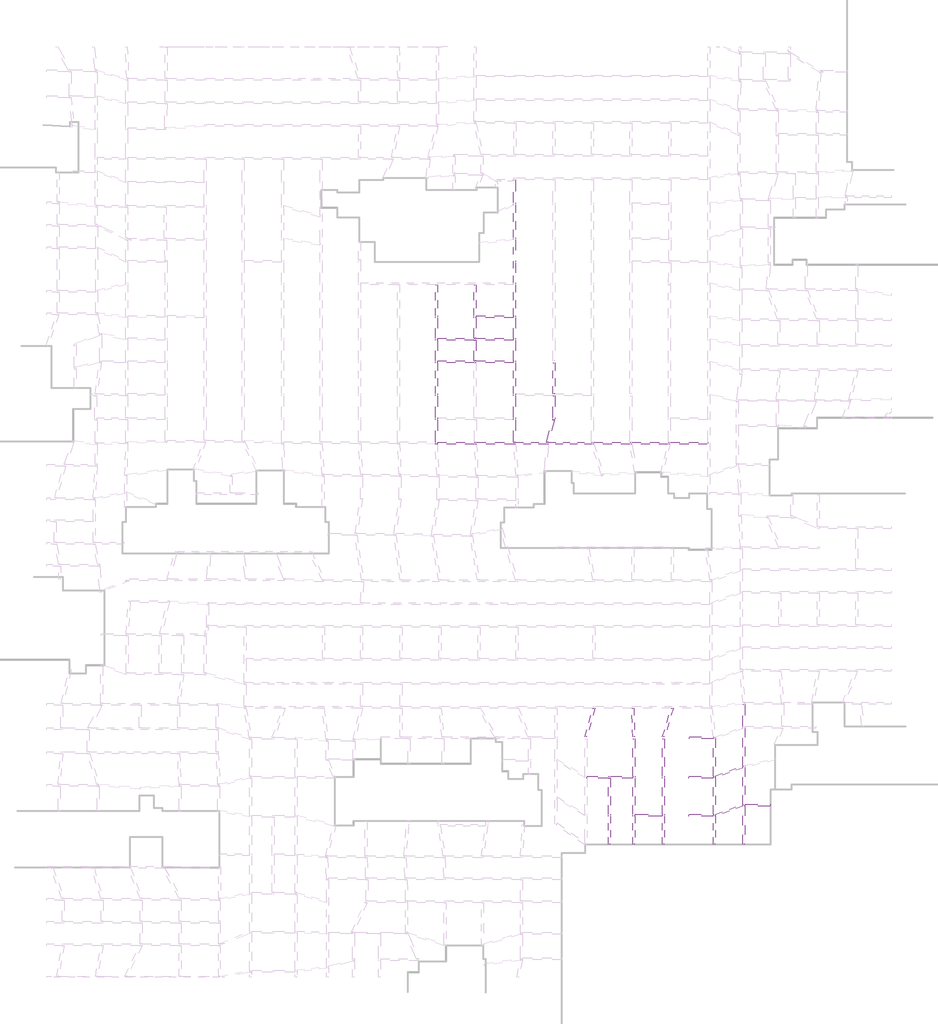
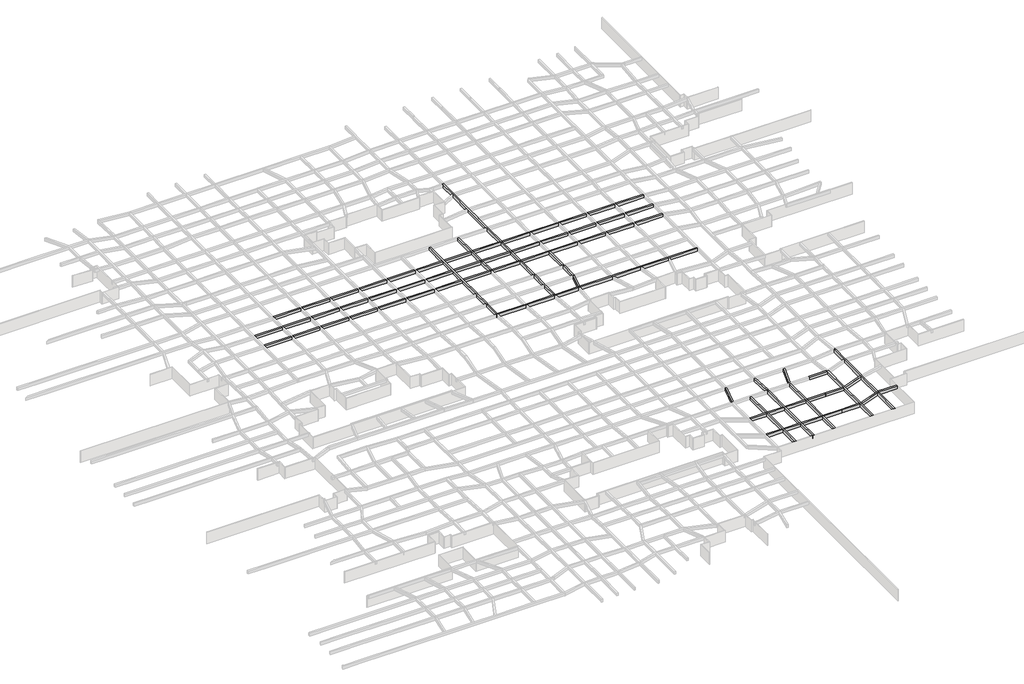
# One storey, part 22 of 45: 27 beams.
"""IFC4 building model written with IfcOpenShell, lengths in millimetres."""

from ifc_helpers import new_model, si_unit, frame, origin, place, context, project, spatial, polyline, outline, extrude, faceted_brep, element, save

model = new_model("IFC4")

# Units and contexts
model_context = context("Model", 3, world=origin())
ifc_project = project(units=[si_unit("LENGTHUNIT", "METRE", prefix="MILLI")], contexts=[model_context])

# Site, building, storey
site = spatial("IfcSite", under=ifc_project)
building = spatial("IfcBuilding", under=site)
storey = spatial("IfcBuildingStorey", under=building, Name="户型图", Elevation=0.0)

# Beams
placement = place(None, origin())
element("IfcBeam", 1, ObjectType="混凝土 - 矩形梁 : KL_beam", at=placement, inside=storey, context=model_context, shape_type="Brep", body=[
    faceted_brep([(-30405.4489038, -29360.4217409, 3300.0), (-30005.4489038, -29360.4217409, 3300.0), (-30005.4489038, -28962.9587641, 3300.0), (-30005.4489038, -24466.2432363, 3300.0), (-30005.4489038, -24066.2432363, 3300.0), (-30005.4489038, -19666.2432363, 3300.0), (-30005.4489038, -19266.2432363, 3300.0), (-30005.4489038, -13006.533538, 3300.0), (-30005.4489038, -12606.533538, 3300.0), (-30005.4489038, -8506.533538, 3300.0), (-30005.4489038, -8106.533538, 3300.0), (-30005.4489038, -3951.5199121, 3300.0), (-30005.4489038, -3551.5199121, 3300.0), (-30005.4489038, 2719.5822838, 3300.0), (-30405.4489038, 2719.5822838, 3300.0), (-30405.4489038, -3551.5199121, 3300.0), (-30405.4489038, -3951.5199121, 3300.0), (-30405.4489038, -8106.533538, 3300.0), (-30405.4489038, -8506.533538, 3300.0), (-30405.4489038, -12606.533538, 3300.0), (-30405.4489038, -13006.533538, 3300.0), (-30405.4489038, -19266.2432363, 3300.0), (-30405.4489038, -19666.2432363, 3300.0), (-30405.4489038, -24066.2432363, 3300.0), (-30405.4489038, -24466.2432363, 3300.0), (-30405.4489038, -28960.389145, 3300.0), (-30405.4489038, -29360.4217409, 2500.0), (-30405.4489038, 2719.5822838, 2500.0), (-30405.4489038, -3551.5199121, 2500.0), (-30405.4489038, -3951.5199121, 2500.0), (-30405.4489038, -8106.533538, 2500.0), (-30405.4489038, -8506.533538, 2500.0), (-30405.4489038, -12606.533538, 2500.0), (-30405.4489038, -13006.533538, 2500.0), (-30405.4489038, -19266.2432363, 2500.0), (-30405.4489038, -19666.2432363, 2500.0), (-30405.4489038, -24066.2432363, 2500.0), (-30405.4489038, -24466.2432363, 2500.0), (-30405.4489038, -28960.389145, 2500.0), (-30005.4489038, -29360.4217409, 2500.0), (-30005.4489038, 2719.5822838, 2500.0), (-30005.4489038, -3551.5199121, 2500.0), (-30005.4489038, -3951.5199121, 2500.0), (-30005.4489038, -8106.533538, 2500.0), (-30005.4489038, -8506.533538, 2500.0), (-30005.4489038, -12606.533538, 2500.0), (-30005.4489038, -13006.533538, 2500.0), (-30005.4489038, -19266.2432363, 2500.0), (-30005.4489038, -19666.2432363, 2500.0), (-30005.4489038, -24066.2432363, 2500.0), (-30005.4489038, -24466.2432363, 2500.0), (-30005.4489038, -28962.9587641, 2500.0)], [[[0, 1, 2, 3, 4, 5, 6, 7, 8, 9, 10, 11, 12, 13, 14, 15, 16, 17, 18, 19, 20, 21, 22, 23, 24, 25]], [[26, 0, 25, 24, 23, 22, 21, 20, 19, 18, 17, 16, 15, 14, 27, 28, 29, 30, 31, 32, 33, 34, 35, 36, 37, 38]], [[39, 26, 38, 37, 36, 35, 34, 33, 32, 31, 30, 29, 28, 27, 40, 41, 42, 43, 44, 45, 46, 47, 48, 49, 50, 51]], [[1, 39, 51, 50, 49, 48, 47, 46, 45, 44, 43, 42, 41, 40, 13, 12, 11, 10, 9, 8, 7, 6, 5, 4, 3, 2]], [[14, 13, 40, 27]], [[1, 0, 26, 39]]]),
])
element("IfcBeam", 2, ObjectType="混凝土 - 矩形梁 : KL_beam", at=placement, inside=storey, context=model_context, shape_type="Brep", body=[
    faceted_brep([(-22249.6349145, 2719.5822838, 3300.0), (-22649.6349145, 2719.5822838, 3300.0), (-22649.6349145, -3551.5199121, 3300.0), (-22649.6349145, -3951.5199121, 3300.0), (-22649.6349145, -8106.533538, 3300.0), (-22249.6349145, -8106.533538, 3300.0), (-22249.6349145, -3951.5199121, 3300.0), (-22249.6349145, -3551.5199121, 3300.0), (-22649.6349145, 2719.5822838, 2500.0), (-22649.6349145, -3551.5199121, 2500.0), (-22649.6349145, -3951.5199121, 2500.0), (-22649.6349145, -8106.533538, 2500.0), (-22249.6349145, 2719.5822838, 2500.0), (-22249.6349145, -3551.5199121, 2500.0), (-22249.6349145, -3951.5199121, 2500.0), (-22249.6349145, -8106.533538, 2500.0)], [[[0, 1, 2, 3, 4, 5, 6, 7]], [[1, 8, 9, 10, 11, 4, 3, 2]], [[8, 12, 13, 14, 15, 11, 10, 9]], [[12, 0, 7, 6, 5, 15, 14, 13]], [[1, 0, 12, 8]], [[5, 4, 11, 15]]]),
])
element("IfcBeam", 3, ObjectType="混凝土 - 矩形梁 : KL_beam", at=placement, inside=storey, context=model_context, shape_type="SweptSolid", body=[
    extrude(outline(polyline([(-22646.4731767, -8506.533538), (-22246.4122455, -8506.533538), (-22174.8464793, -12606.533538), (-22574.9074105, -12606.533538), (-22646.4731767, -8506.533538)])), frame((0.0, 0.0, 2500.0), z_axis=(0.0, 0.0, 1.0), x_axis=(1.0, 0.0, 0.0)), (0.0, 0.0, 1.0), 800.0),
])
element("IfcBeam", 4, ObjectType="混凝土 - 矩形梁 : KL_beam", at=placement, inside=storey, context=model_context, shape_type="Brep", body=[
    faceted_brep([(-14228.2347705, 23868.127427, 3300.0), (-14628.2347705, 23868.127427, 3300.0), (-14628.2347705, 23523.6357489, 3300.0), (-14628.2347705, 19151.8590606, 3300.0), (-14628.2347705, 18698.7467799, 3300.0), (-14628.2347705, 12109.0004081, 3300.0), (-14628.2347705, 11706.0312682, 3300.0), (-14628.2347705, 3119.5822838, 3300.0), (-14628.2347705, 2719.5822838, 3300.0), (-14628.2347705, -3551.5199121, 3300.0), (-14628.2347705, -3951.5199121, 3300.0), (-14628.2347705, -8106.533538, 3300.0), (-14628.2347705, -8506.533538, 3300.0), (-14628.2347705, -12606.533538, 3300.0), (-14628.2347705, -13006.533538, 3300.0), (-14628.2347705, -19266.2432363, 3300.0), (-14628.2347705, -19666.2432363, 3300.0), (-14628.2347705, -24066.2432363, 3300.0), (-14628.2347705, -24466.2432363, 3300.0), (-14628.2347705, -28962.9587641, 3300.0), (-14228.2347705, -28962.9587641, 3300.0), (-14228.2347705, -24466.2432363, 3300.0), (-14228.2347705, -24066.2432363, 3300.0), (-14228.2347705, -19666.2432363, 3300.0), (-14228.2347705, -19266.2432363, 3300.0), (-14228.2347705, -13006.533538, 3300.0), (-14228.2347705, -12606.533538, 3300.0), (-14228.2347705, -8506.533538, 3300.0), (-14228.2347705, -8106.533538, 3300.0), (-14228.2347705, -3951.5199121, 3300.0), (-14228.2347705, -3551.5199121, 3300.0), (-14228.2347705, 2719.5822838, 3300.0), (-14228.2347705, 3119.5822838, 3300.0), (-14228.2347705, 7119.5822838, 3300.0), (-14228.2347705, 7519.5822838, 3300.0), (-14228.2347705, 11731.9876735, 3300.0), (-14228.2347705, 12131.9876735, 3300.0), (-14228.2347705, 18831.9876735, 3300.0), (-14228.2347705, 19231.9876735, 3300.0), (-14628.2347705, 23868.127427, 2500.0), (-14628.2347705, 23523.6357489, 2500.0), (-14628.2347705, 19151.8590606, 2500.0), (-14628.2347705, 18698.7467799, 2500.0), (-14628.2347705, 12109.0004081, 2500.0), (-14628.2347705, 11706.0312682, 2500.0), (-14628.2347705, 3119.5822838, 2500.0), (-14628.2347705, 2719.5822838, 2500.0), (-14628.2347705, -3551.5199121, 2500.0), (-14628.2347705, -3951.5199121, 2500.0), (-14628.2347705, -8106.533538, 2500.0), (-14628.2347705, -8506.533538, 2500.0), (-14628.2347705, -12606.533538, 2500.0), (-14628.2347705, -13006.533538, 2500.0), (-14628.2347705, -19266.2432363, 2500.0), (-14628.2347705, -19666.2432363, 2500.0), (-14628.2347705, -24066.2432363, 2500.0), (-14628.2347705, -24466.2432363, 2500.0), (-14628.2347705, -28962.9587641, 2500.0), (-14228.2347705, 23868.127427, 2500.0), (-14228.2347705, 19231.9876735, 2500.0), (-14228.2347705, 18831.9876735, 2500.0), (-14228.2347705, 12131.9876735, 2500.0), (-14228.2347705, 11731.9876735, 2500.0), (-14228.2347705, 7519.5822838, 2500.0), (-14228.2347705, 7119.5822838, 2500.0), (-14228.2347705, 3119.5822838, 2500.0), (-14228.2347705, 2719.5822838, 2500.0), (-14228.2347705, -3551.5199121, 2500.0), (-14228.2347705, -3951.5199121, 2500.0), (-14228.2347705, -8106.533538, 2500.0), (-14228.2347705, -8506.533538, 2500.0), (-14228.2347705, -12606.533538, 2500.0), (-14228.2347705, -13006.533538, 2500.0), (-14228.2347705, -19266.2432363, 2500.0), (-14228.2347705, -19666.2432363, 2500.0), (-14228.2347705, -24066.2432363, 2500.0), (-14228.2347705, -24466.2432363, 2500.0), (-14228.2347705, -28962.9587641, 2500.0)], [[[0, 1, 2, 3, 4, 5, 6, 7, 8, 9, 10, 11, 12, 13, 14, 15, 16, 17, 18, 19, 20, 21, 22, 23, 24, 25, 26, 27, 28, 29, 30, 31, 32, 33, 34, 35, 36, 37, 38]], [[1, 39, 40, 41, 42, 43, 44, 45, 46, 47, 48, 49, 50, 51, 52, 53, 54, 55, 56, 57, 19, 18, 17, 16, 15, 14, 13, 12, 11, 10, 9, 8, 7, 6, 5, 4, 3, 2]], [[39, 58, 59, 60, 61, 62, 63, 64, 65, 66, 67, 68, 69, 70, 71, 72, 73, 74, 75, 76, 77, 57, 56, 55, 54, 53, 52, 51, 50, 49, 48, 47, 46, 45, 44, 43, 42, 41, 40]], [[58, 0, 38, 37, 36, 35, 34, 33, 32, 31, 30, 29, 28, 27, 26, 25, 24, 23, 22, 21, 20, 77, 76, 75, 74, 73, 72, 71, 70, 69, 68, 67, 66, 65, 64, 63, 62, 61, 60, 59]], [[1, 0, 58, 39]], [[20, 19, 57, 77]]]),
])
element("IfcBeam", 5, ObjectType="混凝土 - 矩形梁 : KL_beam", at=placement, inside=storey, context=model_context, shape_type="SweptSolid", body=[
    extrude(outline(polyline([(-6728.2347705, -13006.533538), (-6328.2347705, -13006.533538), (-6328.2347705, -19266.2432363), (-6728.2347705, -19266.2432363), (-6728.2347705, -13006.533538)])), frame((0.0, 0.0, 2500.0), z_axis=(0.0, 0.0, 1.0), x_axis=(1.0, 0.0, 0.0)), (0.0, 0.0, 1.0), 800.0),
])
element("IfcBeam", 6, ObjectType="混凝土 - 矩形梁 : KL_beam", at=placement, inside=storey, context=model_context, shape_type="Brep", body=[
    faceted_brep([(-6728.2347705, -24466.2432363, 3300.0), (-6375.2608223, -24466.2432363, 3300.0), (-6328.2347705, -24466.2432363, 3300.0), (-6328.2347705, -24066.2432363, 3300.0), (-6328.2347705, -19666.2432363, 3300.0), (-6728.2347705, -19666.2432363, 3300.0), (-6728.2347705, -24066.2432363, 3300.0), (-6728.2347705, -24466.2432363, 2500.0), (-6728.2347705, -19666.2432363, 2500.0), (-6728.2347705, -24066.2432363, 2500.0), (-6328.2347705, -24466.2432363, 2500.0), (-6375.2608223, -24466.2432363, 2500.0), (-6328.2347705, -19666.2432363, 2500.0), (-6328.2347705, -24066.2432363, 2500.0)], [[[0, 1, 2, 3, 4, 5, 6]], [[7, 0, 6, 5, 8, 9]], [[10, 11, 7, 9, 8, 12, 13]], [[2, 10, 13, 12, 4, 3]], [[2, 1, 0, 7, 11, 10]], [[5, 4, 12, 8]]]),
])
element("IfcBeam", 7, ObjectType="混凝土 - 矩形梁 : KL_beam", at=placement, inside=storey, context=model_context, shape_type="SweptSolid", body=[
    extrude(outline(polyline([(-76574.0592951, -3951.5199121), (-76574.0592951, -3551.5199121), (-69259.410716, -3551.5199121), (-69259.410716, -3951.5199121), (-76574.0592951, -3951.5199121)])), frame((0.0, 0.0, 2500.0), z_axis=(0.0, 0.0, 1.0), x_axis=(1.0, 0.0, 0.0)), (0.0, 0.0, 1.0), 800.0),
    extrude(outline(polyline([(24442.7166646, -3551.5199121), (24442.7166646, -3951.5199121), (16905.3597604, -3951.5199121), (16905.3597604, -3551.5199121), (24442.7166646, -3551.5199121)])), frame((0.0, 0.0, 2500.0), z_axis=(0.0, 0.0, 1.0), x_axis=(1.0, 0.0, 0.0)), (0.0, 0.0, 1.0), 800.0),
    extrude(outline(polyline([(-68859.410716, -3951.5199121), (-68859.410716, -3551.5199121), (-61385.2176693, -3551.5199121), (-61385.2176693, -3951.5199121), (-68859.410716, -3951.5199121)])), frame((0.0, 0.0, 2500.0), z_axis=(0.0, 0.0, 1.0), x_axis=(1.0, 0.0, 0.0)), (0.0, 0.0, 1.0), 800.0),
    extrude(outline(polyline([(-60985.2176693, -3951.5199121), (-60985.2176693, -3551.5199121), (-53571.0209029, -3551.5199121), (-53571.0209029, -3951.5199121), (-60985.2176693, -3951.5199121)])), frame((0.0, 0.0, 2500.0), z_axis=(0.0, 0.0, 1.0), x_axis=(1.0, 0.0, 0.0)), (0.0, 0.0, 1.0), 800.0),
    extrude(outline(polyline([(-53171.0209029, -3951.5199121), (-53171.0209029, -3551.5199121), (-45810.5958048, -3551.5199121), (-45810.5958048, -3951.5199121), (-53171.0209029, -3951.5199121)])), frame((0.0, 0.0, 2500.0), z_axis=(0.0, 0.0, 1.0), x_axis=(1.0, 0.0, 0.0)), (0.0, 0.0, 1.0), 800.0),
    extrude(outline(polyline([(-45410.5958048, -3951.5199121), (-45410.5958048, -3551.5199121), (-38013.9760147, -3551.5199121), (-38013.9760147, -3951.5199121), (-45410.5958048, -3951.5199121)])), frame((0.0, 0.0, 2500.0), z_axis=(0.0, 0.0, 1.0), x_axis=(1.0, 0.0, 0.0)), (0.0, 0.0, 1.0), 800.0),
    extrude(outline(polyline([(-37613.9760147, -3951.5199121), (-37613.9760147, -3551.5199121), (-30405.4489038, -3551.5199121), (-30405.4489038, -3951.5199121), (-37613.9760147, -3951.5199121)])), frame((0.0, 0.0, 2500.0), z_axis=(0.0, 0.0, 1.0), x_axis=(1.0, 0.0, 0.0)), (0.0, 0.0, 1.0), 800.0),
    extrude(outline(polyline([(-30005.4489038, -3951.5199121), (-30005.4489038, -3551.5199121), (-22649.6349145, -3551.5199121), (-22649.6349145, -3951.5199121), (-30005.4489038, -3951.5199121)])), frame((0.0, 0.0, 2500.0), z_axis=(0.0, 0.0, 1.0), x_axis=(1.0, 0.0, 0.0)), (0.0, 0.0, 1.0), 800.0),
    extrude(outline(polyline([(-22249.6349145, -3951.5199121), (-22249.6349145, -3551.5199121), (-14628.2347705, -3551.5199121), (-14628.2347705, -3951.5199121), (-22249.6349145, -3951.5199121)])), frame((0.0, 0.0, 2500.0), z_axis=(0.0, 0.0, 1.0), x_axis=(1.0, 0.0, 0.0)), (0.0, 0.0, 1.0), 800.0),
    extrude(outline(polyline([(-14228.2347705, -3951.5199121), (-14228.2347705, -3551.5199121), (-6728.2347705, -3551.5199121), (-6728.2347705, -3951.5199121), (-14228.2347705, -3951.5199121)])), frame((0.0, 0.0, 2500.0), z_axis=(0.0, 0.0, 1.0), x_axis=(1.0, 0.0, 0.0)), (0.0, 0.0, 1.0), 800.0),
    extrude(outline(polyline([(-6328.2347705, -3951.5199121), (-6328.2347705, -3551.5199121), (1071.7652295, -3551.5199121), (1071.7652295, -3951.5199121), (-6328.2347705, -3951.5199121)])), frame((0.0, 0.0, 2500.0), z_axis=(0.0, 0.0, 1.0), x_axis=(1.0, 0.0, 0.0)), (0.0, 0.0, 1.0), 800.0),
    extrude(outline(polyline([(1471.7652295, -3951.5199121), (1471.7652295, -3551.5199121), (8769.3873949, -3551.5199121), (8769.3873949, -3951.5199121), (1471.7652295, -3951.5199121)])), frame((0.0, 0.0, 2500.0), z_axis=(0.0, 0.0, 1.0), x_axis=(1.0, 0.0, 0.0)), (0.0, 0.0, 1.0), 800.0),
    extrude(outline(polyline([(9169.3873949, -3951.5199121), (9169.3873949, -3551.5199121), (16505.3597604, -3551.5199121), (16505.3597604, -3951.5199121), (9169.3873949, -3951.5199121)])), frame((0.0, 0.0, 2500.0), z_axis=(0.0, 0.0, 1.0), x_axis=(1.0, 0.0, 0.0)), (0.0, 0.0, 1.0), 800.0),
])
element("IfcBeam", 8, ObjectType="混凝土 - 矩形梁 : KL_beam", at=placement, inside=storey, context=model_context, shape_type="Brep", body=[
    faceted_brep([(-84386.4058027, -12606.533538, 3300.0), (-84386.4058027, -13006.533538, 3300.0), (-76974.0592951, -13006.533538, 3300.0), (-76974.0592951, -12606.533538, 3300.0), (-84386.4058027, -13006.533538, 2500.0), (-76974.0592951, -13006.533538, 2500.0), (-84386.4058027, -12606.533538, 2500.0), (-76974.0592951, -12606.533538, 2500.0)], [[[0, 1, 2, 3]], [[1, 4, 5, 2]], [[4, 6, 7, 5]], [[6, 0, 3, 7]], [[1, 0, 6, 4]], [[3, 2, 5, 7]]]),
    faceted_brep([(24442.7166646, -12606.533538, 3300.0), (24442.7166646, -13006.533538, 3300.0), (24442.7166646, -13006.533538, 2500.0), (24442.7166646, -12606.533538, 2500.0), (16905.3597604, -13006.533538, 3300.0), (16905.3597604, -12606.533538, 3300.0), (16905.3597604, -12606.533538, 2500.0), (16905.3597604, -13006.533538, 2500.0)], [[[0, 1, 2, 3]], [[4, 5, 6, 7]], [[1, 0, 5, 4]], [[2, 1, 4, 7]], [[3, 2, 7, 6]], [[0, 3, 6, 5]]]),
    faceted_brep([(-76574.0592951, -13006.533538, 3300.0), (-76574.0592951, -12606.533538, 3300.0), (-76574.0592951, -12606.533538, 2500.0), (-76574.0592951, -13006.533538, 2500.0), (-69259.410716, -12606.533538, 3300.0), (-69259.410716, -13006.533538, 3300.0), (-69259.410716, -13006.533538, 2500.0), (-69259.410716, -12606.533538, 2500.0)], [[[0, 1, 2, 3]], [[4, 5, 6, 7]], [[1, 0, 5, 4]], [[0, 3, 6, 5]], [[3, 2, 7, 6]], [[2, 1, 4, 7]]]),
    faceted_brep([(-68859.410716, -12606.533538, 3300.0), (-68859.410716, -13006.533538, 3300.0), (-61385.2176693, -13006.533538, 3300.0), (-61385.2176693, -12606.533538, 3300.0), (-68859.410716, -13006.533538, 2500.0), (-61385.2176693, -13006.533538, 2500.0), (-68859.410716, -12606.533538, 2500.0), (-61385.2176693, -12606.533538, 2500.0)], [[[0, 1, 2, 3]], [[1, 4, 5, 2]], [[4, 6, 7, 5]], [[6, 0, 3, 7]], [[1, 0, 6, 4]], [[3, 2, 5, 7]]]),
    faceted_brep([(-60985.2176693, -13006.533538, 3300.0), (-60985.2176693, -12606.533538, 3300.0), (-60985.2176693, -12606.533538, 2500.0), (-60985.2176693, -13006.533538, 2500.0), (-53571.0209029, -12606.533538, 3300.0), (-53571.0209029, -13006.533538, 3300.0), (-53571.0209029, -13006.533538, 2500.0), (-53571.0209029, -12606.533538, 2500.0)], [[[0, 1, 2, 3]], [[4, 5, 6, 7]], [[1, 0, 5, 4]], [[0, 3, 6, 5]], [[3, 2, 7, 6]], [[2, 1, 4, 7]]]),
    faceted_brep([(-53171.0209029, -12606.533538, 3300.0), (-53171.0209029, -13006.533538, 3300.0), (-45810.5958048, -13006.533538, 3300.0), (-45810.5958048, -12606.533538, 3300.0), (-53171.0209029, -13006.533538, 2500.0), (-45810.5958048, -13006.533538, 2500.0), (-53171.0209029, -12606.533538, 2500.0), (-45810.5958048, -12606.533538, 2500.0)], [[[0, 1, 2, 3]], [[1, 4, 5, 2]], [[4, 6, 7, 5]], [[6, 0, 3, 7]], [[1, 0, 6, 4]], [[3, 2, 5, 7]]]),
    faceted_brep([(-45410.5958048, -13006.533538, 3300.0), (-45410.5958048, -12606.533538, 3300.0), (-45410.5958048, -12606.533538, 2500.0), (-45410.5958048, -13006.533538, 2500.0), (-38013.9760147, -12606.533538, 3300.0), (-38013.9760147, -13006.533538, 3300.0), (-38013.9760147, -13006.533538, 2500.0), (-38013.9760147, -12606.533538, 2500.0)], [[[0, 1, 2, 3]], [[4, 5, 6, 7]], [[1, 0, 5, 4]], [[0, 3, 6, 5]], [[3, 2, 7, 6]], [[2, 1, 4, 7]]]),
    faceted_brep([(-37613.9760147, -12606.533538, 3300.0), (-37613.9760147, -13006.533538, 3300.0), (-30405.4489038, -13006.533538, 3300.0), (-30405.4489038, -12606.533538, 3300.0), (-37613.9760147, -13006.533538, 2500.0), (-30405.4489038, -13006.533538, 2500.0), (-37613.9760147, -12606.533538, 2500.0), (-30405.4489038, -12606.533538, 2500.0)], [[[0, 1, 2, 3]], [[1, 4, 5, 2]], [[4, 6, 7, 5]], [[6, 0, 3, 7]], [[1, 0, 6, 4]], [[3, 2, 5, 7]]]),
    faceted_brep([(-30005.4489038, -13006.533538, 3300.0), (-30005.4489038, -12606.533538, 3300.0), (-30005.4489038, -12606.533538, 2500.0), (-30005.4489038, -13006.533538, 2500.0), (-14628.2347705, -12606.533538, 3300.0), (-14628.2347705, -13006.533538, 3300.0), (-14628.2347705, -13006.533538, 2500.0), (-14628.2347705, -12606.533538, 2500.0), (-22569.0047968, -13006.533538, 3300.0), (-22169.0047968, -13006.533538, 3300.0), (-22174.8464793, -12606.533538, 3300.0), (-22574.9074105, -12606.533538, 3300.0), (-22569.0047968, -13006.533538, 2500.0), (-22169.0047968, -13006.533538, 2500.0), (-22574.9074105, -12606.533538, 2500.0), (-22174.8464793, -12606.533538, 2500.0)], [[[0, 1, 2, 3]], [[4, 5, 6, 7]], [[1, 0, 8, 9, 5, 4, 10, 11]], [[0, 3, 12, 13, 6, 5, 9, 8]], [[3, 2, 14, 15, 7, 6, 13, 12]], [[2, 1, 11, 10, 4, 7, 15, 14]]]),
    faceted_brep([(-14228.2347705, -12606.533538, 3300.0), (-14228.2347705, -13006.533538, 3300.0), (-6728.2347705, -13006.533538, 3300.0), (-6328.2347705, -13006.533538, 3300.0), (1071.7652295, -13006.533538, 3300.0), (1071.7652295, -12606.533538, 3300.0), (-6328.2347705, -12606.533538, 3300.0), (-6728.2347705, -12606.533538, 3300.0), (-14228.2347705, -13006.533538, 2500.0), (-6728.2347705, -13006.533538, 2500.0), (-6328.2347705, -13006.533538, 2500.0), (1071.7652295, -13006.533538, 2500.0), (-14228.2347705, -12606.533538, 2500.0), (-6728.2347705, -12606.533538, 2500.0), (-6328.2347705, -12606.533538, 2500.0), (1071.7652295, -12606.533538, 2500.0)], [[[0, 1, 2, 3, 4, 5, 6, 7]], [[1, 8, 9, 10, 11, 4, 3, 2]], [[8, 12, 13, 14, 15, 11, 10, 9]], [[12, 0, 7, 6, 5, 15, 14, 13]], [[1, 0, 12, 8]], [[5, 4, 11, 15]]]),
    faceted_brep([(1471.7652295, -13006.533538, 3300.0), (1471.7652295, -12606.533538, 3300.0), (1471.7652295, -12606.533538, 2500.0), (1471.7652295, -13006.533538, 2500.0), (8769.3873949, -12606.533538, 3300.0), (8769.3873949, -13006.533538, 3300.0), (8769.3873949, -13006.533538, 2500.0), (8769.3873949, -12606.533538, 2500.0)], [[[0, 1, 2, 3]], [[4, 5, 6, 7]], [[1, 0, 5, 4]], [[0, 3, 6, 5]], [[3, 2, 7, 6]], [[2, 1, 4, 7]]]),
    faceted_brep([(9169.3873949, -12606.533538, 3300.0), (9169.3873949, -13006.533538, 3300.0), (16505.3597604, -13006.533538, 3300.0), (16505.3597604, -12606.533538, 3300.0), (9169.3873949, -13006.533538, 2500.0), (16505.3597604, -13006.533538, 2500.0), (9169.3873949, -12606.533538, 2500.0), (16505.3597604, -12606.533538, 2500.0)], [[[0, 1, 2, 3]], [[1, 4, 5, 2]], [[4, 6, 7, 5]], [[6, 0, 3, 7]], [[1, 0, 6, 4]], [[3, 2, 5, 7]]]),
])
element("IfcBeam", 9, ObjectType="混凝土 - 矩形梁 : KL_beam", at=placement, inside=storey, context=model_context, shape_type="Brep", body=[
    faceted_brep([(24442.7166646, -8506.533538, 3300.0), (24442.7166646, -8106.533538, 3300.0), (16905.3597604, -8106.533538, 3300.0), (16905.3597604, -8506.533538, 3300.0), (24442.7166646, -8106.533538, 2500.0), (16905.3597604, -8106.533538, 2500.0), (24442.7166646, -8506.533538, 2500.0), (16905.3597604, -8506.533538, 2500.0)], [[[0, 1, 2, 3]], [[1, 4, 5, 2]], [[4, 6, 7, 5]], [[6, 0, 3, 7]], [[1, 0, 6, 4]], [[3, 2, 5, 7]]]),
    faceted_brep([(-84386.4058027, -8506.533538, 3300.0), (-84386.4058027, -8106.533538, 3300.0), (-84386.4058027, -8106.533538, 2500.0), (-84386.4058027, -8506.533538, 2500.0), (-76974.0592951, -8106.533538, 3300.0), (-76974.0592951, -8506.533538, 3300.0), (-76974.0592951, -8506.533538, 2500.0), (-76974.0592951, -8106.533538, 2500.0)], [[[0, 1, 2, 3]], [[4, 5, 6, 7]], [[1, 0, 5, 4]], [[2, 1, 4, 7]], [[3, 2, 7, 6]], [[0, 3, 6, 5]]]),
    faceted_brep([(-76574.0592951, -8506.533538, 3300.0), (-76574.0592951, -8106.533538, 3300.0), (-76574.0592951, -8106.533538, 2500.0), (-76574.0592951, -8506.533538, 2500.0), (-69259.410716, -8106.533538, 3300.0), (-69259.410716, -8506.533538, 3300.0), (-69259.410716, -8506.533538, 2500.0), (-69259.410716, -8106.533538, 2500.0)], [[[0, 1, 2, 3]], [[4, 5, 6, 7]], [[1, 0, 5, 4]], [[2, 1, 4, 7]], [[3, 2, 7, 6]], [[0, 3, 6, 5]]]),
    faceted_brep([(-68859.410716, -8506.533538, 3300.0), (-68859.410716, -8106.533538, 3300.0), (-68859.410716, -8106.533538, 2500.0), (-68859.410716, -8506.533538, 2500.0), (-61385.2176693, -8106.533538, 3300.0), (-61385.2176693, -8506.533538, 3300.0), (-61385.2176693, -8506.533538, 2500.0), (-61385.2176693, -8106.533538, 2500.0)], [[[0, 1, 2, 3]], [[4, 5, 6, 7]], [[1, 0, 5, 4]], [[2, 1, 4, 7]], [[3, 2, 7, 6]], [[0, 3, 6, 5]]]),
    faceted_brep([(-60985.2176693, -8506.533538, 3300.0), (-60985.2176693, -8106.533538, 3300.0), (-60985.2176693, -8106.533538, 2500.0), (-60985.2176693, -8506.533538, 2500.0), (-53571.0209029, -8106.533538, 3300.0), (-53571.0209029, -8506.533538, 3300.0), (-53571.0209029, -8506.533538, 2500.0), (-53571.0209029, -8106.533538, 2500.0)], [[[0, 1, 2, 3]], [[4, 5, 6, 7]], [[1, 0, 5, 4]], [[2, 1, 4, 7]], [[3, 2, 7, 6]], [[0, 3, 6, 5]]]),
    faceted_brep([(-53171.0209029, -8506.533538, 3300.0), (-53171.0209029, -8106.533538, 3300.0), (-53171.0209029, -8106.533538, 2500.0), (-53171.0209029, -8506.533538, 2500.0), (-45810.5958048, -8106.533538, 3300.0), (-45810.5958048, -8506.533538, 3300.0), (-45810.5958048, -8506.533538, 2500.0), (-45810.5958048, -8106.533538, 2500.0)], [[[0, 1, 2, 3]], [[4, 5, 6, 7]], [[1, 0, 5, 4]], [[2, 1, 4, 7]], [[3, 2, 7, 6]], [[0, 3, 6, 5]]]),
    faceted_brep([(-45410.5958048, -8506.533538, 3300.0), (-45410.5958048, -8106.533538, 3300.0), (-45410.5958048, -8106.533538, 2500.0), (-45410.5958048, -8506.533538, 2500.0), (-38013.9760147, -8106.533538, 3300.0), (-38013.9760147, -8506.533538, 3300.0), (-38013.9760147, -8506.533538, 2500.0), (-38013.9760147, -8106.533538, 2500.0)], [[[0, 1, 2, 3]], [[4, 5, 6, 7]], [[1, 0, 5, 4]], [[2, 1, 4, 7]], [[3, 2, 7, 6]], [[0, 3, 6, 5]]]),
    faceted_brep([(-37613.9760147, -8506.533538, 3300.0), (-37613.9760147, -8106.533538, 3300.0), (-37613.9760147, -8106.533538, 2500.0), (-37613.9760147, -8506.533538, 2500.0), (-30405.4489038, -8106.533538, 3300.0), (-30405.4489038, -8506.533538, 3300.0), (-30405.4489038, -8506.533538, 2500.0), (-30405.4489038, -8106.533538, 2500.0)], [[[0, 1, 2, 3]], [[4, 5, 6, 7]], [[1, 0, 5, 4]], [[2, 1, 4, 7]], [[3, 2, 7, 6]], [[0, 3, 6, 5]]]),
    faceted_brep([(-30005.4489038, -8506.533538, 3300.0), (-30005.4489038, -8106.533538, 3300.0), (-30005.4489038, -8106.533538, 2500.0), (-30005.4489038, -8506.533538, 2500.0), (-14628.2347705, -8106.533538, 3300.0), (-14628.2347705, -8506.533538, 3300.0), (-14628.2347705, -8506.533538, 2500.0), (-14628.2347705, -8106.533538, 2500.0), (-22646.4731767, -8506.533538, 3300.0), (-22246.4122455, -8506.533538, 3300.0), (-22249.6349145, -8106.533538, 3300.0), (-22649.6349145, -8106.533538, 3300.0), (-22249.6349145, -8106.533538, 2500.0), (-22649.6349145, -8106.533538, 2500.0), (-22246.4122455, -8506.533538, 2500.0), (-22646.4731767, -8506.533538, 2500.0)], [[[0, 1, 2, 3]], [[4, 5, 6, 7]], [[1, 0, 8, 9, 5, 4, 10, 11]], [[2, 1, 11, 10, 4, 7, 12, 13]], [[3, 2, 13, 12, 7, 6, 14, 15]], [[0, 3, 15, 14, 6, 5, 9, 8]]]),
    faceted_brep([(-14228.2347705, -8506.533538, 3300.0), (-14228.2347705, -8106.533538, 3300.0), (-14228.2347705, -8106.533538, 2500.0), (-14228.2347705, -8506.533538, 2500.0), (-6728.2347705, -8106.533538, 3300.0), (-6728.2347705, -8506.533538, 3300.0), (-6728.2347705, -8506.533538, 2500.0), (-6728.2347705, -8106.533538, 2500.0)], [[[0, 1, 2, 3]], [[4, 5, 6, 7]], [[1, 0, 5, 4]], [[2, 1, 4, 7]], [[3, 2, 7, 6]], [[0, 3, 6, 5]]]),
    faceted_brep([(-6328.2347705, -8506.533538, 3300.0), (-6328.2347705, -8106.533538, 3300.0), (-6328.2347705, -8106.533538, 2500.0), (-6328.2347705, -8506.533538, 2500.0), (1071.7652295, -8106.533538, 3300.0), (1071.7652295, -8506.533538, 3300.0), (1071.7652295, -8506.533538, 2500.0), (1071.7652295, -8106.533538, 2500.0)], [[[0, 1, 2, 3]], [[4, 5, 6, 7]], [[1, 0, 5, 4]], [[2, 1, 4, 7]], [[3, 2, 7, 6]], [[0, 3, 6, 5]]]),
    faceted_brep([(1471.7652295, -8506.533538, 3300.0), (1471.7652295, -8106.533538, 3300.0), (1471.7652295, -8106.533538, 2500.0), (1471.7652295, -8506.533538, 2500.0), (8769.3873949, -8106.533538, 3300.0), (8769.3873949, -8506.533538, 3300.0), (8769.3873949, -8506.533538, 2500.0), (8769.3873949, -8106.533538, 2500.0)], [[[0, 1, 2, 3]], [[4, 5, 6, 7]], [[1, 0, 5, 4]], [[2, 1, 4, 7]], [[3, 2, 7, 6]], [[0, 3, 6, 5]]]),
    faceted_brep([(9169.3873949, -8506.533538, 3300.0), (9169.3873949, -8106.533538, 3300.0), (9169.3873949, -8106.533538, 2500.0), (9169.3873949, -8506.533538, 2500.0), (16505.3597604, -8106.533538, 3300.0), (16505.3597604, -8506.533538, 3300.0), (16505.3597604, -8506.533538, 2500.0), (16505.3597604, -8106.533538, 2500.0)], [[[0, 1, 2, 3]], [[4, 5, 6, 7]], [[1, 0, 5, 4]], [[2, 1, 4, 7]], [[3, 2, 7, 6]], [[0, 3, 6, 5]]]),
])
element("IfcBeam", 10, ObjectType="混凝土 - 矩形梁 : KL_beam", at=placement, inside=storey, context=model_context, shape_type="Brep", body=[
    faceted_brep([(-30005.4489038, -28962.9587641, 3300.0), (-30005.4489038, -29360.4217409, 3300.0), (-30005.4489038, -29362.9587641, 3300.0), (-29994.7663876, -29362.9587641, 3300.0), (-22513.251878, -29362.9587641, 3300.0), (-22112.7029396, -29362.9587641, 3300.0), (-14615.089027, -29362.9587641, 3300.0), (-14214.1641855, -29362.9587641, 3300.0), (-8055.2383922, -29362.9587641, 3300.0), (-7654.2726844, -29362.9587641, 3300.0), (1123.7861901, -29362.9587641, 3300.0), (1542.0628927, -29362.9587641, 3300.0), (8798.6279221, -29362.9587641, 3300.0), (9203.6139724, -29362.9587641, 3300.0), (16448.7904357, -29362.9587641, 3300.0), (16861.2162982, -29362.9587641, 3300.0), (24442.7166646, -29362.9587641, 3300.0), (24442.7166646, -28962.9587641, 3300.0), (16905.3597604, -28962.9587641, 3300.0), (16505.3597604, -28962.9587641, 3300.0), (9169.3873949, -28962.9587641, 3300.0), (8769.3873949, -28962.9587641, 3300.0), (1471.7652295, -28962.9587641, 3300.0), (1071.7652295, -28962.9587641, 3300.0), (-7580.1521166, -28962.9587641, 3300.0), (-7994.2625887, -28962.9587641, 3300.0), (-14228.2347705, -28962.9587641, 3300.0), (-14628.2347705, -28962.9587641, 3300.0), (-22123.4502387, -28962.9587641, 3300.0), (-22523.4502387, -28962.9587641, 3300.0), (-30005.4489038, -29362.9587641, 2500.0), (-29994.7663876, -29362.9587641, 2500.0), (-22513.251878, -29362.9587641, 2500.0), (-22112.7029396, -29362.9587641, 2500.0), (-14615.089027, -29362.9587641, 2500.0), (-14214.1641855, -29362.9587641, 2500.0), (-8055.2383922, -29362.9587641, 2500.0), (-7654.2726844, -29362.9587641, 2500.0), (1123.7861901, -29362.9587641, 2500.0), (1542.0628927, -29362.9587641, 2500.0), (8798.6279221, -29362.9587641, 2500.0), (9203.6139724, -29362.9587641, 2500.0), (16448.7904357, -29362.9587641, 2500.0), (16861.2162982, -29362.9587641, 2500.0), (24442.7166646, -29362.9587641, 2500.0), (-30005.4489038, -29360.4217409, 2500.0), (-30005.4489038, -28962.9587641, 2500.0), (-22523.4502387, -28962.9587641, 2500.0), (-22123.4502387, -28962.9587641, 2500.0), (-14628.2347705, -28962.9587641, 2500.0), (-14228.2347705, -28962.9587641, 2500.0), (-7994.2625887, -28962.9587641, 2500.0), (-7580.1521166, -28962.9587641, 2500.0), (1071.7652295, -28962.9587641, 2500.0), (1471.7652295, -28962.9587641, 2500.0), (8769.3873949, -28962.9587641, 2500.0), (9169.3873949, -28962.9587641, 2500.0), (16505.3597604, -28962.9587641, 2500.0), (16905.3597604, -28962.9587641, 2500.0), (24442.7166646, -28962.9587641, 2500.0)], [[[0, 1, 2, 3, 4, 5, 6, 7, 8, 9, 10, 11, 12, 13, 14, 15, 16, 17, 18, 19, 20, 21, 22, 23, 24, 25, 26, 27, 28, 29]], [[2, 30, 31, 32, 33, 34, 35, 36, 37, 38, 39, 40, 41, 42, 43, 44, 16, 15, 14, 13, 12, 11, 10, 9, 8, 7, 6, 5, 4, 3]], [[30, 45, 46, 47, 48, 49, 50, 51, 52, 53, 54, 55, 56, 57, 58, 59, 44, 43, 42, 41, 40, 39, 38, 37, 36, 35, 34, 33, 32, 31]], [[46, 0, 29, 28, 27, 26, 25, 24, 23, 22, 21, 20, 19, 18, 17, 59, 58, 57, 56, 55, 54, 53, 52, 51, 50, 49, 48, 47]], [[0, 46, 45, 30, 2, 1]], [[17, 16, 44, 59]]]),
])
element("IfcBeam", 11, ObjectType="混凝土 - 矩形梁 : KL_beam", at=placement, inside=storey, context=model_context, shape_type="Brep", body=[
    faceted_brep([(-7994.2625887, -28962.9587641, 2500.0), (-7994.2625887, -28962.9587641, 3300.0), (-6789.3712945, -24466.2432363, 3300.0), (-6789.3712945, -24466.2432363, 2500.0), (-7580.1521166, -28962.9587641, 3300.0), (-7580.1521166, -28962.9587641, 2500.0), (-6728.2347705, -24466.2432363, 3300.0), (-6375.2608223, -24466.2432363, 3300.0), (-6375.2608223, -24466.2432363, 2500.0), (-6728.2347705, -24466.2432363, 2500.0)], [[[0, 1, 2, 3]], [[4, 1, 0, 5]], [[3, 2, 6, 7, 8, 9]], [[1, 4, 7, 6, 2]], [[5, 0, 3, 9, 8]], [[4, 5, 8, 7]]]),
])
element("IfcBeam", 12, ObjectType="混凝土 - 矩形梁 : KL_beam", at=placement, inside=storey, context=model_context, shape_type="Brep", body=[
    faceted_brep([(31916.4740744, -109927.8268455, 3300.0), (31516.4740744, -109927.8268455, 3300.0), (31516.4740744, -109927.8268455, 2500.0), (31916.4740744, -109927.8268455, 2500.0), (31916.4740744, -102188.0123265, 3300.0), (31916.4740744, -101788.0123265, 3300.0), (31916.4740744, -94427.0995098, 3300.0), (31916.4740744, -94016.5778667, 3300.0), (31916.4740744, -86494.0851447, 3300.0), (31916.4740744, -86094.0851447, 3300.0), (31916.4740744, -81717.9371223, 3300.0), (31916.4740744, -81694.8851233, 3300.0), (31516.4740744, -81743.9989477, 3300.0), (31516.4740744, -86246.4848419, 3300.0), (31516.4740744, -86671.1120245, 3300.0), (31516.4740744, -94126.9529942, 3300.0), (31516.4740744, -94551.5801768, 3300.0), (31516.4740744, -101846.9529942, 3300.0), (31516.4740744, -102271.5801768, 3300.0), (31516.4740744, -81743.9989477, 2500.0), (31516.4740744, -86246.4848419, 2500.0), (31516.4740744, -86671.1120245, 2500.0), (31516.4740744, -94126.9529942, 2500.0), (31516.4740744, -94551.5801768, 2500.0), (31516.4740744, -101846.9529942, 2500.0), (31516.4740744, -102271.5801768, 2500.0), (31916.4740744, -81694.8851233, 2500.0), (31916.4740744, -81717.9371223, 2500.0), (31916.4740744, -86094.0851447, 2500.0), (31916.4740744, -86494.0851447, 2500.0), (31916.4740744, -94016.5778667, 2500.0), (31916.4740744, -94427.0995098, 2500.0), (31916.4740744, -101788.0123265, 2500.0), (31916.4740744, -102188.0123265, 2500.0)], [[[0, 1, 2, 3]], [[1, 0, 4, 5, 6, 7, 8, 9, 10, 11, 12, 13, 14, 15, 16, 17, 18]], [[2, 1, 18, 17, 16, 15, 14, 13, 12, 19, 20, 21, 22, 23, 24, 25]], [[3, 2, 25, 24, 23, 22, 21, 20, 19, 26, 27, 28, 29, 30, 31, 32, 33]], [[0, 3, 33, 32, 31, 30, 29, 28, 27, 26, 11, 10, 9, 8, 7, 6, 5, 4]], [[11, 26, 19, 12]]]),
    faceted_brep([(31916.4740744, -81317.9371223, 3300.0), (31916.4740744, -81317.9371223, 2500.0), (31900.9194594, -81317.9371223, 2500.0), (31900.9194594, -81317.9371223, 3300.0), (31916.4740744, -81509.5363909, 3300.0), (31916.4740744, -81509.5363909, 2500.0)], [[[0, 1, 2, 3]], [[4, 3, 2, 5]], [[4, 0, 3]], [[1, 5, 2]], [[1, 0, 4, 5]]]),
])
element("IfcBeam", 13, ObjectType="混凝土 - 矩形梁 : KL_beam", at=placement, inside=storey, context=model_context, shape_type="SweptSolid", body=[
    extrude(outline(polyline([(37059.476209, -101788.0123265), (37059.476209, -102188.0123265), (31916.4740744, -102188.0123265), (31916.4740744, -101788.0123265), (37059.476209, -101788.0123265)])), frame((0.0, 0.0, 2500.0), z_axis=(0.0, 0.0, 1.0), x_axis=(1.0, 0.0, 0.0)), (0.0, 0.0, 1.0), 800.0),
])
element("IfcBeam", 14, ObjectType="混凝土 - 矩形梁 : KL_beam", at=placement, inside=storey, context=model_context, shape_type="Brep", body=[
    faceted_brep([(26022.028798, -109927.9389906, 3300.0), (25622.028798, -109927.9389906, 3300.0), (25622.028798, -109927.9389906, 2500.0), (26022.028798, -109927.9389906, 2500.0), (26022.028798, -104229.0724192, 3300.0), (26022.028798, -103804.4452366, 3300.0), (26022.028798, -96509.0724192, 3300.0), (26022.028798, -96084.4452366, 3300.0), (26022.028798, -88628.6042669, 3300.0), (26022.028798, -88475.6331307, 3300.0), (25622.028798, -88500.0981788, 3300.0), (25622.028798, -88687.9389906, 3300.0), (25622.028798, -96168.0123265, 3300.0), (25622.028798, -96568.0123265, 3300.0), (25622.028798, -103888.0123265, 3300.0), (25622.028798, -104288.0123265, 3300.0), (25622.028798, -88500.0981788, 2500.0), (25622.028798, -88687.9389906, 2500.0), (25622.028798, -96168.0123265, 2500.0), (25622.028798, -96568.0123265, 2500.0), (25622.028798, -103888.0123265, 2500.0), (25622.028798, -104288.0123265, 2500.0), (26022.028798, -88475.6331307, 2500.0), (26022.028798, -88628.6042669, 2500.0), (26022.028798, -96084.4452366, 2500.0), (26022.028798, -96509.0724192, 2500.0), (26022.028798, -103804.4452366, 2500.0), (26022.028798, -104229.0724192, 2500.0)], [[[0, 1, 2, 3]], [[1, 0, 4, 5, 6, 7, 8, 9, 10, 11, 12, 13, 14, 15]], [[2, 1, 15, 14, 13, 12, 11, 10, 16, 17, 18, 19, 20, 21]], [[3, 2, 21, 20, 19, 18, 17, 16, 22, 23, 24, 25, 26, 27]], [[0, 3, 27, 26, 25, 24, 23, 22, 9, 8, 7, 6, 5, 4]], [[9, 22, 16, 10]]]),
])
element("IfcBeam", 15, ObjectType="混凝土 - 矩形梁 : KL_beam", at=placement, inside=storey, context=model_context, shape_type="SweptSolid", body=[
    extrude(outline(polyline([(25622.028798, -88687.9389906), (20722.028798, -88687.9389906), (20722.028798, -88287.9389906), (25595.9789252, -88287.9389906), (25622.028798, -88500.0981788), (25622.028798, -88687.9389906)])), frame((0.0, 0.0, 2500.0), z_axis=(0.0, 0.0, 1.0), x_axis=(1.0, 0.0, 0.0)), (0.0, 0.0, 1.0), 800.0),
])
element("IfcBeam", 16, ObjectType="混凝土 - 矩形梁 : KL_beam", at=placement, inside=storey, context=model_context, shape_type="SweptSolid", body=[
    extrude(outline(polyline([(20622.028798, -96568.0123265), (20622.028798, -96168.0123265), (25622.028798, -96168.0123265), (25622.028798, -96568.0123265), (20622.028798, -96568.0123265)])), frame((0.0, 0.0, 2500.0), z_axis=(0.0, 0.0, 1.0), x_axis=(1.0, 0.0, 0.0)), (0.0, 0.0, 1.0), 800.0),
])
element("IfcBeam", 17, ObjectType="混凝土 - 矩形梁 : KL_beam", at=placement, inside=storey, context=model_context, shape_type="SweptSolid", body=[
    extrude(outline(polyline([(20622.028798, -104288.0123265), (20622.028798, -103888.0123265), (25622.028798, -103888.0123265), (25622.028798, -104288.0123265), (20622.028798, -104288.0123265)])), frame((0.0, 0.0, 2500.0), z_axis=(0.0, 0.0, 1.0), x_axis=(1.0, 0.0, 0.0)), (0.0, 0.0, 1.0), 800.0),
])
element("IfcBeam", 18, ObjectType="混凝土 - 矩形梁 : KL_beam", at=placement, inside=storey, context=model_context, shape_type="SweptSolid", body=[
    extrude(outline(polyline([(31516.4740744, -101846.9529942), (31516.4740744, -102271.5801768), (26022.028798, -104229.0724192), (26022.028798, -103804.4452366), (31516.4740744, -101846.9529942)])), frame((0.0, 0.0, 2500.0), z_axis=(0.0, 0.0, 1.0), x_axis=(1.0, 0.0, 0.0)), (0.0, 0.0, 1.0), 800.0),
])
element("IfcBeam", 19, ObjectType="混凝土 - 矩形梁 : KL_beam", at=placement, inside=storey, context=model_context, shape_type="SweptSolid", body=[
    extrude(outline(polyline([(31516.4740744, -94126.9529942), (31516.4740744, -94551.5801768), (26022.028798, -96509.0724192), (26022.028798, -96084.4452366), (31516.4740744, -94126.9529942)])), frame((0.0, 0.0, 2500.0), z_axis=(0.0, 0.0, 1.0), x_axis=(1.0, 0.0, 0.0)), (0.0, 0.0, 1.0), 800.0),
])
element("IfcBeam", 20, ObjectType="混凝土 - 矩形梁 : KL_beam", at=placement, inside=storey, context=model_context, shape_type="SweptSolid", body=[
    extrude(outline(polyline([(1277.3669177, -82534.4617231), (1691.4773898, -82534.4617231), (149.8378023, -88287.9389906), (-264.2726698, -88287.9389906), (1277.3669177, -82534.4617231)])), frame((0.0, 0.0, 2500.0), z_axis=(0.0, 0.0, 1.0), x_axis=(1.0, 0.0, 0.0)), (0.0, 0.0, 1.0), 800.0),
])
element("IfcBeam", 21, ObjectType="混凝土 - 矩形梁 : KL_beam", at=placement, inside=storey, context=model_context, shape_type="SweptSolid", body=[
    extrude(outline(polyline([(9144.8742373, -82534.4617231), (9545.118055, -82534.4617231), (9746.0339084, -88287.9389906), (9345.7900907, -88287.9389906), (9144.8742373, -82534.4617231)])), frame((0.0, 0.0, 2500.0), z_axis=(0.0, 0.0, 1.0), x_axis=(1.0, 0.0, 0.0)), (0.0, 0.0, 1.0), 800.0),
])
element("IfcBeam", 22, ObjectType="混凝土 - 矩形梁 : KL_beam", at=placement, inside=storey, context=model_context, shape_type="SweptSolid", body=[
    extrude(outline(polyline([(17090.3022302, -82534.4617231), (17508.5789328, -82534.4617231), (15749.5644071, -88287.9389906), (15331.2877045, -88287.9389906), (17090.3022302, -82534.4617231)])), frame((0.0, 0.0, 2500.0), z_axis=(0.0, 0.0, 1.0), x_axis=(1.0, 0.0, 0.0)), (0.0, 0.0, 1.0), 800.0),
])
element("IfcBeam", 23, ObjectType="混凝土 - 矩形梁 : KL_beam", at=placement, inside=storey, context=model_context, shape_type="Brep", body=[
    faceted_brep([(9752.8961535, -109927.9756585, 3300.0), (9352.8961535, -109927.9756585, 3300.0), (9352.8961535, -109927.9756585, 2500.0), (9752.8961535, -109927.9756585, 2500.0), (9752.8961535, -104288.0123265, 3300.0), (9752.8961535, -103888.0123265, 3300.0), (9752.8961535, -96568.0123265, 3300.0), (9752.8961535, -96168.0123265, 3300.0), (9752.8961535, -88687.9389906, 3300.0), (9352.8961535, -88687.9389906, 3300.0), (9352.8961535, -96168.0123265, 3300.0), (9352.8961535, -96568.0123265, 3300.0), (9352.8961535, -103888.0123265, 3300.0), (9352.8961535, -104288.0123265, 3300.0), (9352.8961535, -88687.9389906, 2500.0), (9352.8961535, -96168.0123265, 2500.0), (9352.8961535, -96568.0123265, 2500.0), (9352.8961535, -103888.0123265, 2500.0), (9352.8961535, -104288.0123265, 2500.0), (9752.8961535, -88687.9389906, 2500.0), (9752.8961535, -96168.0123265, 2500.0), (9752.8961535, -96568.0123265, 2500.0), (9752.8961535, -103888.0123265, 2500.0), (9752.8961535, -104288.0123265, 2500.0)], [[[0, 1, 2, 3]], [[1, 0, 4, 5, 6, 7, 8, 9, 10, 11, 12, 13]], [[2, 1, 13, 12, 11, 10, 9, 14, 15, 16, 17, 18]], [[3, 2, 18, 17, 16, 15, 14, 19, 20, 21, 22, 23]], [[0, 3, 23, 22, 21, 20, 19, 8, 7, 6, 5, 4]], [[9, 8, 19, 14]]]),
])
element("IfcBeam", 24, ObjectType="混凝土 - 矩形梁 : KL_beam", at=placement, inside=storey, context=model_context, shape_type="Brep", body=[
    faceted_brep([(15679.3735446, -109927.9756585, 3300.0), (15279.3735446, -109927.9756585, 3300.0), (15279.3735446, -109927.9756585, 2500.0), (15679.3735446, -109927.9756585, 2500.0), (15679.3735446, -104288.0123265, 3300.0), (15679.3735446, -103888.0123265, 3300.0), (15679.3735446, -96568.0123265, 3300.0), (15679.3735446, -96168.0123265, 3300.0), (15679.3735446, -88687.9389906, 3300.0), (15279.3735446, -88687.9389906, 3300.0), (15279.3735446, -96168.0123265, 3300.0), (15279.3735446, -96568.0123265, 3300.0), (15279.3735446, -103888.0123265, 3300.0), (15279.3735446, -104288.0123265, 3300.0), (15279.3735446, -88687.9389906, 2500.0), (15279.3735446, -96168.0123265, 2500.0), (15279.3735446, -96568.0123265, 2500.0), (15279.3735446, -103888.0123265, 2500.0), (15279.3735446, -104288.0123265, 2500.0), (15679.3735446, -88687.9389906, 2500.0), (15679.3735446, -96168.0123265, 2500.0), (15679.3735446, -96568.0123265, 2500.0), (15679.3735446, -103888.0123265, 2500.0), (15679.3735446, -104288.0123265, 2500.0)], [[[0, 1, 2, 3]], [[1, 0, 4, 5, 6, 7, 8, 9, 10, 11, 12, 13]], [[2, 1, 13, 12, 11, 10, 9, 14, 15, 16, 17, 18]], [[3, 2, 18, 17, 16, 15, 14, 19, 20, 21, 22, 23]], [[0, 3, 23, 22, 21, 20, 19, 8, 7, 6, 5, 4]], [[9, 8, 19, 14]]]),
])
element("IfcBeam", 25, ObjectType="混凝土 - 矩形梁 : KL_beam", at=placement, inside=storey, context=model_context, shape_type="Brep", body=[
    faceted_brep([(20622.028798, -96568.0123265, 3300.0), (20622.028798, -96168.0123265, 3300.0), (15679.3735446, -96168.0123265, 3300.0), (15679.3735446, -96568.0123265, 3300.0), (20622.028798, -96168.0123265, 2500.0), (15679.3735446, -96168.0123265, 2500.0), (20622.028798, -96568.0123265, 2500.0), (15679.3735446, -96568.0123265, 2500.0)], [[[0, 1, 2, 3]], [[1, 4, 5, 2]], [[4, 6, 7, 5]], [[6, 0, 3, 7]], [[0, 6, 4, 1]], [[3, 2, 5, 7]]]),
    faceted_brep([(9352.8961535, -96168.0123265, 3300.0), (9352.8961535, -96568.0123265, 3300.0), (9352.8961535, -96568.0123265, 2500.0), (9352.8961535, -96168.0123265, 2500.0), (4889.1927278, -96168.0123265, 3300.0), (4489.1927278, -96168.0123265, 3300.0), (89.1927278, -96168.0123265, 3300.0), (89.1927278, -96568.0123265, 3300.0), (4489.1927278, -96568.0123265, 3300.0), (4889.1927278, -96568.0123265, 3300.0), (4889.1927278, -96168.0123265, 2500.0), (4489.1927278, -96168.0123265, 2500.0), (89.1927278, -96168.0123265, 2500.0), (4889.1927278, -96568.0123265, 2500.0), (4489.1927278, -96568.0123265, 2500.0), (89.1927278, -96568.0123265, 2500.0)], [[[0, 1, 2, 3]], [[1, 0, 4, 5, 6, 7, 8, 9]], [[0, 3, 10, 11, 12, 6, 5, 4]], [[3, 2, 13, 14, 15, 12, 11, 10]], [[2, 1, 9, 8, 7, 15, 14, 13]], [[7, 6, 12, 15]]]),
    faceted_brep([(9752.8961535, -96568.0123265, 3300.0), (9752.8961535, -96168.0123265, 3300.0), (9752.8961535, -96168.0123265, 2500.0), (9752.8961535, -96568.0123265, 2500.0), (15279.3735446, -96168.0123265, 3300.0), (15279.3735446, -96568.0123265, 3300.0), (15279.3735446, -96568.0123265, 2500.0), (15279.3735446, -96168.0123265, 2500.0)], [[[0, 1, 2, 3]], [[4, 5, 6, 7]], [[1, 0, 5, 4]], [[2, 1, 4, 7]], [[3, 2, 7, 6]], [[0, 3, 6, 5]]]),
])
element("IfcBeam", 26, ObjectType="混凝土 - 矩形梁 : KL_beam", at=placement, inside=storey, context=model_context, shape_type="Brep", body=[
    faceted_brep([(4889.1927278, -109927.9756585, 3300.0), (4489.1927278, -109927.9756585, 3300.0), (4489.1927278, -109927.9756585, 2500.0), (4889.1927278, -109927.9756585, 2500.0), (4889.1927278, -104288.0123265, 3300.0), (4889.1927278, -103888.0123265, 3300.0), (4889.1927278, -96568.0123265, 3300.0), (4489.1927278, -96568.0123265, 3300.0), (4489.1927278, -103888.0123265, 3300.0), (4489.1927278, -104288.0123265, 3300.0), (4489.1927278, -96568.0123265, 2500.0), (4489.1927278, -103888.0123265, 2500.0), (4489.1927278, -104288.0123265, 2500.0), (4889.1927278, -96568.0123265, 2500.0), (4889.1927278, -103888.0123265, 2500.0), (4889.1927278, -104288.0123265, 2500.0)], [[[0, 1, 2, 3]], [[1, 0, 4, 5, 6, 7, 8, 9]], [[2, 1, 9, 8, 7, 10, 11, 12]], [[3, 2, 12, 11, 10, 13, 14, 15]], [[0, 3, 15, 14, 13, 6, 5, 4]], [[7, 6, 13, 10]]]),
    faceted_brep([(4489.1927278, -88687.9389906, 3300.0), (4889.1927278, -88687.9389906, 3300.0), (4889.1927278, -88687.9389906, 2500.0), (4489.1927278, -88687.9389906, 2500.0), (4889.1927278, -96168.0123265, 3300.0), (4489.1927278, -96168.0123265, 3300.0), (4489.1927278, -96168.0123265, 2500.0), (4889.1927278, -96168.0123265, 2500.0)], [[[0, 1, 2, 3]], [[4, 5, 6, 7]], [[1, 0, 5, 4]], [[0, 3, 6, 5]], [[3, 2, 7, 6]], [[2, 1, 4, 7]]]),
])
element("IfcBeam", 27, ObjectType="混凝土 - 矩形梁 : KL_beam", at=placement, inside=storey, context=model_context, shape_type="SweptSolid", body=[
    extrude(outline(polyline([(89.1927278, -104288.0123265), (89.1927278, -103888.0123265), (4489.1927278, -103888.0123265), (4489.1927278, -104288.0123265), (89.1927278, -104288.0123265)])), frame((0.0, 0.0, 2500.0), z_axis=(0.0, 0.0, 1.0), x_axis=(1.0, 0.0, 0.0)), (0.0, 0.0, 1.0), 800.0),
    extrude(outline(polyline([(20622.028798, -103888.0123265), (20622.028798, -104288.0123265), (15679.3735446, -104288.0123265), (15679.3735446, -103888.0123265), (20622.028798, -103888.0123265)])), frame((0.0, 0.0, 2500.0), z_axis=(0.0, 0.0, 1.0), x_axis=(1.0, 0.0, 0.0)), (0.0, 0.0, 1.0), 800.0),
    extrude(outline(polyline([(9352.8961535, -103888.0123265), (9352.8961535, -104288.0123265), (4889.1927278, -104288.0123265), (4889.1927278, -103888.0123265), (9352.8961535, -103888.0123265)])), frame((0.0, 0.0, 2500.0), z_axis=(0.0, 0.0, 1.0), x_axis=(1.0, 0.0, 0.0)), (0.0, 0.0, 1.0), 800.0),
    extrude(outline(polyline([(9752.8961535, -104288.0123265), (9752.8961535, -103888.0123265), (15279.3735446, -103888.0123265), (15279.3735446, -104288.0123265), (9752.8961535, -104288.0123265)])), frame((0.0, 0.0, 2500.0), z_axis=(0.0, 0.0, 1.0), x_axis=(1.0, 0.0, 0.0)), (0.0, 0.0, 1.0), 800.0),
])

save(model, "model.ifc")

# Revit data of these elements
# Type "混凝土 - 矩形梁 : KL_beam"
#   Length [instance default] = 1524 mm
#   b = 400 mm
#   h = 800 mm
#   Structural Material [instance default] = 混凝土 - 现场浇注混凝土
#   Assembly Code = ""
# Elements 1, 2, 3, 4, 5, 6, 7, 8, 9, 10, 11, 12, 13, 14, 15, 16, 17, 18, 19, 20, 21, 22, 23, 24, 25, 26, 27 (IfcBeam, "混凝土 - 矩形梁 : KL_beam")
#   Comments = ""
#   Structural Material = none
#   Phase Created = 新构造
# Materials
#   "混凝土 - 现场浇注混凝土": class "混凝土", colour RGB 192 192 192, transparency 0
